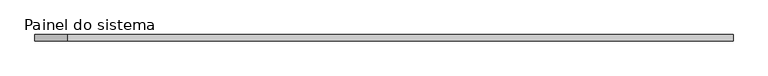
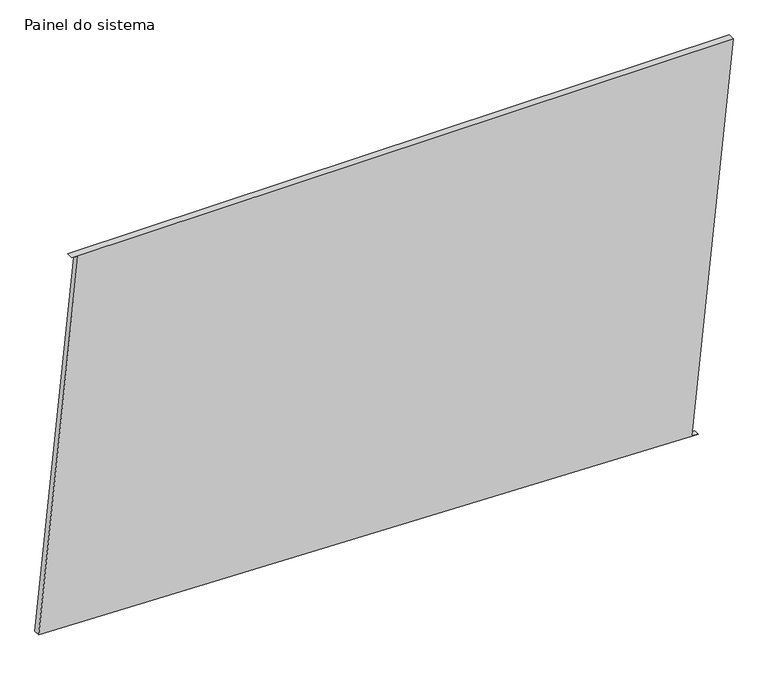
"""IFC4 building model written with IfcOpenShell, lengths in millimetres: plate geometry, Painel do sistema : Envidraçado."""

from ifc_helpers import new_model, si_unit, frame, origin, place, context, project, spatial, polyline, outline, extrude, source, transform, mapped, element, save


def painel_do_sistema_3c39de95(model_context):
    return source(origin(), model_context, "Body", "SweptSolid", [
        extrude(outline(polyline([(0.0, 1209.2454021), (2.5300763, 1184.3737573), (1572.5166616, 1344.0811623), (1572.5166616, -1216.6953373), (1569.9865853, -1191.8236926), (73.2357927, -1344.0811623), (0.0, 1209.2454021)])), frame((0.0, 24.5, 0.0), z_axis=(0.0, 1.0, 0.0), x_axis=(0.0, 0.0, 1.0)), (0.0, 0.0, 1.0), 25.0),
    ])


if __name__ == "__main__":
    model = new_model("IFC4")
    model_context = context("Model", 3, world=origin())
    ifc_project = project(units=[si_unit("LENGTHUNIT", "METRE", prefix="MILLI")], contexts=[model_context])
    site = spatial("IfcSite", under=ifc_project)
    building = spatial("IfcBuilding", under=site)
    placement = place(None, origin())
    painel_do_sistema_shape = painel_do_sistema_3c39de95(model_context)
    element("IfcPlate", 1, ObjectType="Painel do sistema : Envidraçado", at=placement, inside=building, context=model_context, shape_type="MappedRepresentation", body=[
        mapped(painel_do_sistema_shape, transform((0.0, 0.0, 0.0), x_axis=(1.0, 0.0, 0.0), y_axis=(0.0, 1.0, 0.0), z_axis=(0.0, 0.0, 1.0))),
    ])
    save(model, "model.ifc")

# Revit data of these elements
# Type "Painel do sistema : Envidraçado"
#   Construction Type Id = "GSP4R"
#   Analytic Construction = "Vidraça única Pilkington 1/8 pol"
#   Visual Light Transmittance = 0.9
#   Solar Heat Gain Coefficient = 0.86
#   Heat Transfer Coefficient (U) = 6.7069 W/(m²·K)
# Element 1 (IfcPlate, "Painel do sistema : Envidraçado")
#   Materials on its faces: "Vidro"
# Materials
#   "Vidro": class "Vidro", colour RGB 0 128 192, transparency 0.9, Description = "Vidro de sílica", Cost = 0
